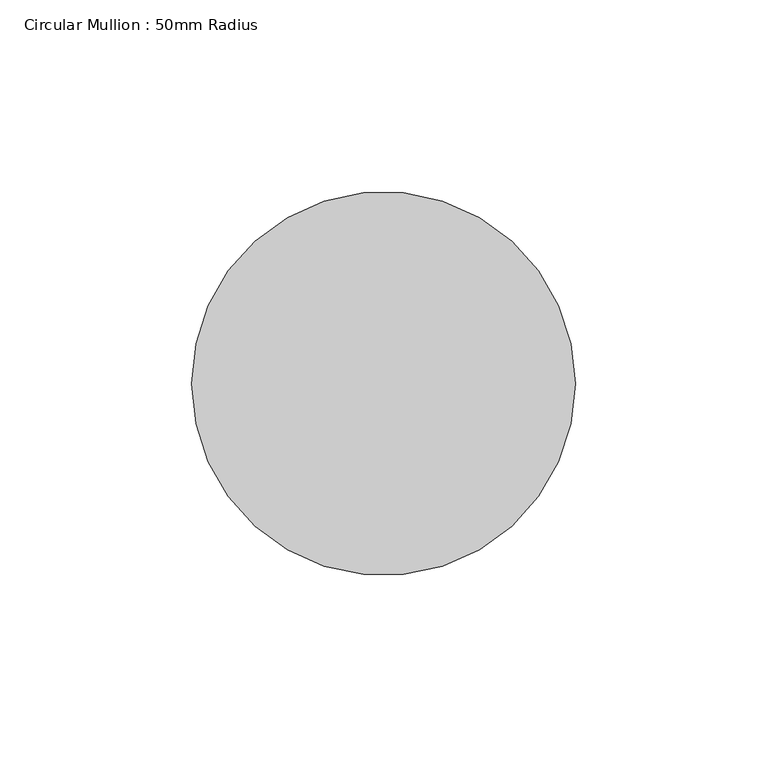
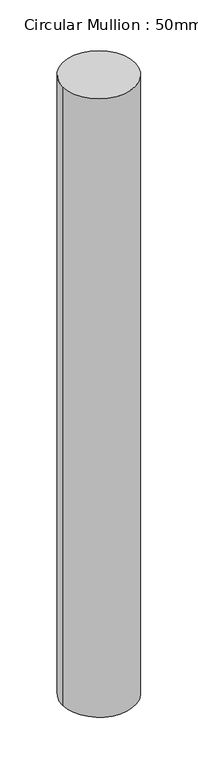
"""IFC4 building model written with IfcOpenShell, lengths in millimetres: member geometry, Circular Mullion : 50mm Radius."""

from ifc_helpers import new_model, si_unit, point, frame, origin, origin_2d, place, context, project, spatial, circle_curve, trimmed, segment, composite_curve, outline, extrude, source, transform, mapped, element, save


def circular_mullion_50mm_radius_fa96ff19(model_context):
    return source(origin(), model_context, "Body", "SweptSolid", [
        extrude(outline(composite_curve([segment(trimmed(circle_curve(origin_2d(), 50.0), [point((50.0, 0.0))], [point((-50.0, 0.0))], False, "CARTESIAN"), True, "CONTINUOUS"), segment(trimmed(circle_curve(origin_2d(), 50.0), [point((-50.0, 0.0))], [point((50.0, 0.0))], False, "CARTESIAN"), True, "CONTINUOUS")], self_intersect=False)), frame((0.0, 0.0, -901.3622864), z_axis=(0.0, 0.0, 1.0), x_axis=(1.0, 0.0, 0.0)), (0.0, 0.0, 1.0), 901.3622864),
    ])


if __name__ == "__main__":
    model = new_model("IFC4")
    model_context = context("Model", 3, world=origin())
    ifc_project = project(units=[si_unit("LENGTHUNIT", "METRE", prefix="MILLI")], contexts=[model_context])
    site = spatial("IfcSite", under=ifc_project)
    building = spatial("IfcBuilding", under=site)
    placement = place(None, origin())
    circular_mullion_50mm_radius_shape = circular_mullion_50mm_radius_fa96ff19(model_context)
    element("IfcMember", 1, ObjectType="Circular Mullion : 50mm Radius", at=placement, inside=building, context=model_context, shape_type="MappedRepresentation", body=[
        mapped(circular_mullion_50mm_radius_shape, transform((0.0, 0.0, 0.0), x_axis=(1.0, 0.0, 0.0), y_axis=(0.0, 1.0, 0.0), z_axis=(0.0, 0.0, 1.0))),
    ])
    save(model, "model.ifc")

# Revit data of these elements
# Type "Circular Mullion : 50mm Radius"
#   built-in parameter 1007350 = 0.164042 (stored number, unit not read)
# Element 1 (IfcMember, "Circular Mullion : 50mm Radius")
#   Materials on its faces: "Aluminium"
# Materials
#   "Aluminium": class "Metal", colour RGB 247 247 247, transparency 0, Description = "Aluminium 6061", Cost = 0
